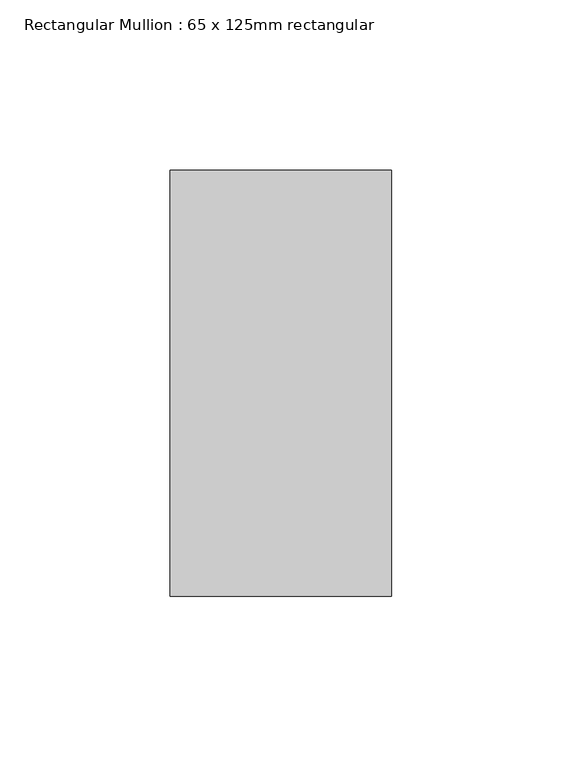
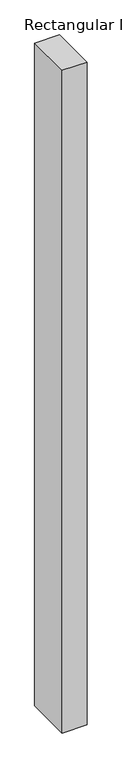
"""IFC4 building model written with IfcOpenShell, lengths in millimetres: member geometry, Rectangular Mullion : 65 x 125mm rectangular."""

import ifcopenshell
import ifcopenshell.guid

model = None  # the IFC model being written
_history = None  # IfcOwnerHistory: only IFC2X3 demands one
_inside = {}  # id of a spatial element -> (the spatial element, [elements in it])
_under = {}  # id of a project, library or spatial element -> (it, [spatial elements below it])
_declared = {}  # id of a project -> (the project, [libraries it declares])
_typed = {}  # id of a type object -> (the type object, [elements of that type])
_made_of = {}  # id of a material, layer set ... -> (it, [elements and type objects made of it])


def new_model(schema):
    """Start an empty IFC model of exactly this schema.

    Asked for "IFC4X3", IfcOpenShell would pick the latest addendum, in which some entities
    have other attributes; the version numbers below select the first issue.
    IFC2X3 requires an IfcOwnerHistory on every rooted entity: one is made here for all.
    """
    global model, _history
    if schema == "IFC4X3":
        model = ifcopenshell.file(schema_version=(4, 3, 0, 0))
    else:
        model = ifcopenshell.file(schema=schema)
    _inside.clear()
    _under.clear()
    _declared.clear()
    _typed.clear()
    _made_of.clear()
    _history = None
    if model.schema == "IFC2X3":
        org = make("IfcOrganization", Name="unknown")
        user = make(
            "IfcPersonAndOrganization",
            ThePerson=make("IfcPerson", FamilyName="unknown"),
            TheOrganization=org,
        )
        app = make(
            "IfcApplication",
            ApplicationDeveloper=org,
            Version="unknown",
            ApplicationFullName="unknown",
            ApplicationIdentifier="unknown",
        )
        _history = make(
            "IfcOwnerHistory",
            OwningUser=user,
            OwningApplication=app,
            ChangeAction="ADDED",
            CreationDate=0,
        )
    return model


def make(cls, **values):
    """One entity of the class cls with the attributes given. An attribute that is None is left unset."""
    return model.create_entity(
        cls, **{name: value for name, value in values.items() if value is not None}
    )


def rooted(cls, **values):
    """An entity with a GlobalId (a new one), such as an element, a storey or a relation."""
    return make(cls, GlobalId=ifcopenshell.guid.new(), OwnerHistory=_history, **values)


def si_unit(unit_type, name, prefix=None):
    """IfcSIUnit, for example si_unit("LENGTHUNIT", "METRE", prefix="MILLI")."""
    return make("IfcSIUnit", UnitType=unit_type, Prefix=prefix, Name=name)


def assignment(units):
    """IfcUnitAssignment: the units of a project."""
    return None if units is None else make("IfcUnitAssignment", Units=units)


def point(xyz):
    """IfcCartesianPoint."""
    return None if xyz is None else make("IfcCartesianPoint", Coordinates=xyz)


def direction(xyz):
    """IfcDirection."""
    return None if xyz is None else make("IfcDirection", DirectionRatios=xyz)


def frame(location, z_axis=None, x_axis=None):
    """IfcAxis2Placement3D, a coordinate frame: its origin and axes. An axis left out is left unset."""
    return make(
        "IfcAxis2Placement3D",
        Location=point(location),
        Axis=direction(z_axis),
        RefDirection=direction(x_axis),
    )


def origin():
    """The frame at (0, 0, 0) with its axes left unset."""
    return frame((0.0, 0.0, 0.0))


def place(relative_to, where):
    """IfcLocalPlacement: puts the frame where relative to a parent placement (None: the world)."""
    return make(
        "IfcLocalPlacement", PlacementRelTo=relative_to, RelativePlacement=where
    )


def context(
    kind, dimensions, precision=None, world=None, true_north=None, identifier=None
):
    """IfcGeometricRepresentationContext, for example the 3D "Model" context."""
    return make(
        "IfcGeometricRepresentationContext",
        ContextIdentifier=identifier,
        ContextType=kind,
        CoordinateSpaceDimension=dimensions,
        Precision=precision,
        WorldCoordinateSystem=world,
        TrueNorth=true_north,
    )


def project(units=None, contexts=None):
    """IfcProject with its units and contexts."""
    return rooted(
        "IfcProject",
        Name="project",
        RepresentationContexts=contexts,
        UnitsInContext=assignment(units),
    )


def spatial(cls, under=None, at=None, **own):
    """A site, building, storey or space (cls), placed at a placement, below another one or the project."""
    s = rooted(cls, ObjectPlacement=at, **own)
    if under is not None:
        _under.setdefault(under.id(), (under, []))[1].append(s)
    return s


def polyline(points):
    """IfcPolyline through the points."""
    return make("IfcPolyline", Points=[point(p) for p in points])


def outline(outer, holes=None, kind="AREA"):
    """IfcArbitraryClosedProfileDef: a profile drawn as a closed curve; with holes, ...WithVoids."""
    if holes is None:
        return make("IfcArbitraryClosedProfileDef", ProfileType=kind, OuterCurve=outer)
    return make(
        "IfcArbitraryProfileDefWithVoids",
        ProfileType=kind,
        OuterCurve=outer,
        InnerCurves=holes,
    )


def extrude(swept, where, along, depth):
    """IfcExtrudedAreaSolid: the profile swept, set in the frame where, extruded along a direction by depth."""
    return make(
        "IfcExtrudedAreaSolid",
        SweptArea=swept,
        Position=where,
        ExtrudedDirection=direction(along),
        Depth=depth,
    )


def shape(context_of_items, identifier, shape_type, items):
    """IfcShapeRepresentation: the items that make up one representation, for example the "Body"."""
    return make(
        "IfcShapeRepresentation",
        ContextOfItems=context_of_items,
        RepresentationIdentifier=identifier,
        RepresentationType=shape_type,
        Items=items,
    )


def source(mapping_origin, context_of_items, identifier, shape_type, items):
    """IfcRepresentationMap: a shape defined once, which mapped items show again and again."""
    return make(
        "IfcRepresentationMap",
        MappingOrigin=mapping_origin,
        MappedRepresentation=shape(context_of_items, identifier, shape_type, items),
    )


def transform(
    local_origin,
    x_axis=None,
    y_axis=None,
    z_axis=None,
    scale=None,
    scale2=None,
    scale3=None,
    uniform=True,
):
    """IfcCartesianTransformationOperator3D, or its non-uniform kind. x_axis, y_axis, z_axis: its Axis1, 2, 3."""
    if uniform:
        return make(
            "IfcCartesianTransformationOperator3D",
            Axis1=direction(x_axis),
            Axis2=direction(y_axis),
            LocalOrigin=point(local_origin),
            Scale=scale,
            Axis3=direction(z_axis),
        )
    return make(
        "IfcCartesianTransformationOperator3DnonUniform",
        Axis1=direction(x_axis),
        Axis2=direction(y_axis),
        LocalOrigin=point(local_origin),
        Scale=scale,
        Axis3=direction(z_axis),
        Scale2=scale2,
        Scale3=scale3,
    )


def mapped(mapping_source, mapping_target):
    """IfcMappedItem: shows the shape of a source again, moved by a transform."""
    return make(
        "IfcMappedItem", MappingSource=mapping_source, MappingTarget=mapping_target
    )


def made_of(thing, what):
    """Note that an element or type object is made of a material, layer set ...; save() writes the relation."""
    if what is not None:
        _made_of.setdefault(what.id(), (what, []))[1].append(thing)
    return thing


def element(
    cls,
    number,
    at=None,
    inside=None,
    cuts=None,
    type_object=None,
    material=None,
    context=None,
    identifier="Body",
    shape_type=None,
    held_by="IfcProductDefinitionShape",
    body=None,
    shapes=None,
    **own,
):
    """One element of the class cls, such as IfcWall. Its Tag is "e" and its number.

    at: its placement. inside: the storey or other place that contains it. cuts: it is an
    opening in that element (IfcRelVoidsElement). A single representation is given by context,
    identifier, shape_type and body (its items); several are given by shapes. held_by: the class
    of the entity that holds the representations. save() writes the other relations.
    """
    e = rooted(cls, Tag="e%d" % number, ObjectPlacement=at, **own)
    if body is not None:
        shapes = [shape(context, identifier, shape_type, body)]
    if shapes is not None:
        e.Representation = make(held_by, Representations=shapes)
    if inside is not None:
        _inside.setdefault(inside.id(), (inside, []))[1].append(e)
    if cuts is not None:
        rooted(
            "IfcRelVoidsElement", RelatingBuildingElement=cuts, RelatedOpeningElement=e
        )
    if type_object is not None:
        _typed.setdefault(type_object.id(), (type_object, []))[1].append(e)
    return made_of(e, material)


def aggregate(whole, parts):
    """IfcRelAggregates: a whole, such as a stair, and the parts it consists of."""
    return rooted("IfcRelAggregates", RelatingObject=whole, RelatedObjects=parts)


def save(model, path):
    """Write the relations noted so far, then the file.

    IfcRelAggregates (storeys below a building ...), IfcRelContainedInSpatialStructure (elements
    in a storey), IfcRelDefinesByType, IfcRelAssociatesMaterial and IfcRelDeclares: one each for
    every whole, place, type object, material and project.
    """
    for whole, parts in _under.values():
        aggregate(whole, parts)
    for where, things in _inside.values():
        rooted(
            "IfcRelContainedInSpatialStructure",
            RelatedElements=things,
            RelatingStructure=where,
        )
    for kind, things in _typed.values():
        rooted("IfcRelDefinesByType", RelatedObjects=things, RelatingType=kind)
    for what, things in _made_of.values():
        rooted("IfcRelAssociatesMaterial", RelatedObjects=things, RelatingMaterial=what)
    for by, libraries in _declared.values():
        rooted("IfcRelDeclares", RelatingContext=by, RelatedDefinitions=libraries)
    model.write(path)


def rectangular_mullion_65_x_125mm_rectangular_c7ba065f(model_context):
    return source(origin(), model_context, "Body", "SweptSolid", [
        extrude(outline(polyline([(0.0, 62.5), (0.0, -62.5), (-65.0, -62.5), (-65.0, 62.5), (0.0, 62.5)])), frame((0.0, 0.0, -1841.6666665), z_axis=(0.0, 0.0, 1.0), x_axis=(1.0, 0.0, 0.0)), (0.0, 0.0, 1.0), 1841.6666665),
    ])


if __name__ == "__main__":
    model = new_model("IFC4")
    model_context = context("Model", 3, world=origin())
    ifc_project = project(units=[si_unit("LENGTHUNIT", "METRE", prefix="MILLI")], contexts=[model_context])
    site = spatial("IfcSite", under=ifc_project)
    building = spatial("IfcBuilding", under=site)
    placement = place(None, origin())
    rectangular_mullion_65_x_125mm_rectangular_shape = rectangular_mullion_65_x_125mm_rectangular_c7ba065f(model_context)
    element("IfcMember", 1, ObjectType="Rectangular Mullion : 65 x 125mm rectangular", at=placement, inside=building, context=model_context, shape_type="MappedRepresentation", body=[
        mapped(rectangular_mullion_65_x_125mm_rectangular_shape, transform((0.0, 0.0, 0.0), x_axis=(1.0, 0.0, 0.0), y_axis=(0.0, 1.0, 0.0), z_axis=(0.0, 0.0, 1.0))),
    ])
    save(model, "model.ifc")

# Revit data of these elements
# Type "Rectangular Mullion : 65 x 125mm rectangular"
#   built-in parameter 1007304 = 0.410105 (stored number, unit not read)
#   built-in parameter 1007301 = 0.106627 (stored number, unit not read)
#   built-in parameter 1007300 = 0.106627 (stored number, unit not read)
# Element 1 (IfcMember, "Rectangular Mullion : 65 x 125mm rectangular")
#   Materials on its faces: "Aluminum"
# Materials
#   "Aluminum": class "Metal", colour RGB 244 245 246, transparency 0, Description = "Aluminum 6061", Cost = 0
